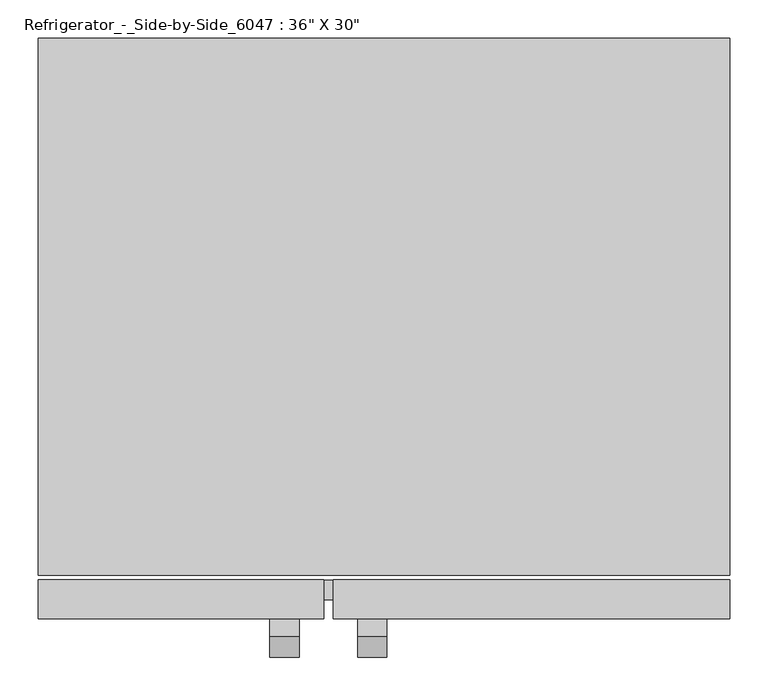
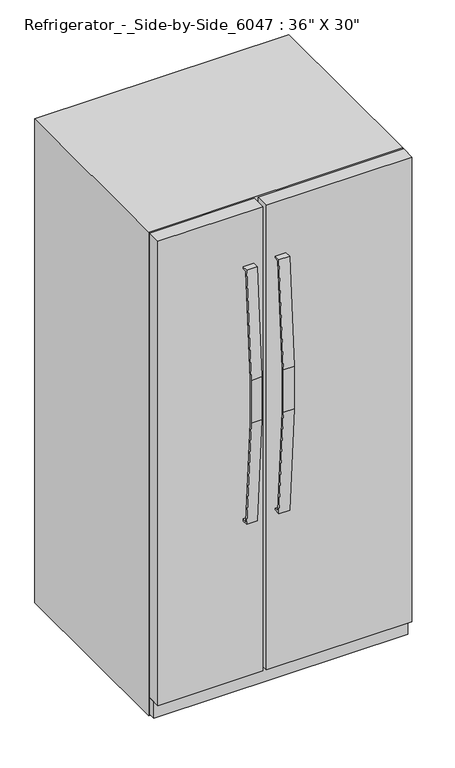
"""IFC4 building model written with IfcOpenShell, lengths in millimetres: proxy geometry."""

import ifcopenshell
import ifcopenshell.guid

model = None  # the IFC model being written
_history = None  # IfcOwnerHistory: only IFC2X3 demands one
_inside = {}  # id of a spatial element -> (the spatial element, [elements in it])
_under = {}  # id of a project, library or spatial element -> (it, [spatial elements below it])
_declared = {}  # id of a project -> (the project, [libraries it declares])
_typed = {}  # id of a type object -> (the type object, [elements of that type])
_made_of = {}  # id of a material, layer set ... -> (it, [elements and type objects made of it])


def new_model(schema):
    """Start an empty IFC model of exactly this schema.

    Asked for "IFC4X3", IfcOpenShell would pick the latest addendum, in which some entities
    have other attributes; the version numbers below select the first issue.
    IFC2X3 requires an IfcOwnerHistory on every rooted entity: one is made here for all.
    """
    global model, _history
    if schema == "IFC4X3":
        model = ifcopenshell.file(schema_version=(4, 3, 0, 0))
    else:
        model = ifcopenshell.file(schema=schema)
    _inside.clear()
    _under.clear()
    _declared.clear()
    _typed.clear()
    _made_of.clear()
    _history = None
    if model.schema == "IFC2X3":
        org = make("IfcOrganization", Name="unknown")
        user = make(
            "IfcPersonAndOrganization",
            ThePerson=make("IfcPerson", FamilyName="unknown"),
            TheOrganization=org,
        )
        app = make(
            "IfcApplication",
            ApplicationDeveloper=org,
            Version="unknown",
            ApplicationFullName="unknown",
            ApplicationIdentifier="unknown",
        )
        _history = make(
            "IfcOwnerHistory",
            OwningUser=user,
            OwningApplication=app,
            ChangeAction="ADDED",
            CreationDate=0,
        )
    return model


def make(cls, **values):
    """One entity of the class cls with the attributes given. An attribute that is None is left unset."""
    return model.create_entity(
        cls, **{name: value for name, value in values.items() if value is not None}
    )


def rooted(cls, **values):
    """An entity with a GlobalId (a new one), such as an element, a storey or a relation."""
    return make(cls, GlobalId=ifcopenshell.guid.new(), OwnerHistory=_history, **values)


def si_unit(unit_type, name, prefix=None):
    """IfcSIUnit, for example si_unit("LENGTHUNIT", "METRE", prefix="MILLI")."""
    return make("IfcSIUnit", UnitType=unit_type, Prefix=prefix, Name=name)


def assignment(units):
    """IfcUnitAssignment: the units of a project."""
    return None if units is None else make("IfcUnitAssignment", Units=units)


def point(xyz):
    """IfcCartesianPoint."""
    return None if xyz is None else make("IfcCartesianPoint", Coordinates=xyz)


def direction(xyz):
    """IfcDirection."""
    return None if xyz is None else make("IfcDirection", DirectionRatios=xyz)


def frame(location, z_axis=None, x_axis=None):
    """IfcAxis2Placement3D, a coordinate frame: its origin and axes. An axis left out is left unset."""
    return make(
        "IfcAxis2Placement3D",
        Location=point(location),
        Axis=direction(z_axis),
        RefDirection=direction(x_axis),
    )


def origin():
    """The frame at (0, 0, 0) with its axes left unset."""
    return frame((0.0, 0.0, 0.0))


def origin_with_axes():
    """The frame at (0, 0, 0) with the z axis (0, 0, 1) and the x axis (1, 0, 0) written out."""
    return frame((0.0, 0.0, 0.0), z_axis=(0.0, 0.0, 1.0), x_axis=(1.0, 0.0, 0.0))


def place(relative_to, where):
    """IfcLocalPlacement: puts the frame where relative to a parent placement (None: the world)."""
    return make(
        "IfcLocalPlacement", PlacementRelTo=relative_to, RelativePlacement=where
    )


def context(
    kind, dimensions, precision=None, world=None, true_north=None, identifier=None
):
    """IfcGeometricRepresentationContext, for example the 3D "Model" context."""
    return make(
        "IfcGeometricRepresentationContext",
        ContextIdentifier=identifier,
        ContextType=kind,
        CoordinateSpaceDimension=dimensions,
        Precision=precision,
        WorldCoordinateSystem=world,
        TrueNorth=true_north,
    )


def project(units=None, contexts=None):
    """IfcProject with its units and contexts."""
    return rooted(
        "IfcProject",
        Name="project",
        RepresentationContexts=contexts,
        UnitsInContext=assignment(units),
    )


def spatial(cls, under=None, at=None, **own):
    """A site, building, storey or space (cls), placed at a placement, below another one or the project."""
    s = rooted(cls, ObjectPlacement=at, **own)
    if under is not None:
        _under.setdefault(under.id(), (under, []))[1].append(s)
    return s


def polyline(points):
    """IfcPolyline through the points."""
    return make("IfcPolyline", Points=[point(p) for p in points])


def outline(outer, holes=None, kind="AREA"):
    """IfcArbitraryClosedProfileDef: a profile drawn as a closed curve; with holes, ...WithVoids."""
    if holes is None:
        return make("IfcArbitraryClosedProfileDef", ProfileType=kind, OuterCurve=outer)
    return make(
        "IfcArbitraryProfileDefWithVoids",
        ProfileType=kind,
        OuterCurve=outer,
        InnerCurves=holes,
    )


def extrude(swept, where, along, depth):
    """IfcExtrudedAreaSolid: the profile swept, set in the frame where, extruded along a direction by depth."""
    return make(
        "IfcExtrudedAreaSolid",
        SweptArea=swept,
        Position=where,
        ExtrudedDirection=direction(along),
        Depth=depth,
    )


def shape(context_of_items, identifier, shape_type, items):
    """IfcShapeRepresentation: the items that make up one representation, for example the "Body"."""
    return make(
        "IfcShapeRepresentation",
        ContextOfItems=context_of_items,
        RepresentationIdentifier=identifier,
        RepresentationType=shape_type,
        Items=items,
    )


def source(mapping_origin, context_of_items, identifier, shape_type, items):
    """IfcRepresentationMap: a shape defined once, which mapped items show again and again."""
    return make(
        "IfcRepresentationMap",
        MappingOrigin=mapping_origin,
        MappedRepresentation=shape(context_of_items, identifier, shape_type, items),
    )


def transform(
    local_origin,
    x_axis=None,
    y_axis=None,
    z_axis=None,
    scale=None,
    scale2=None,
    scale3=None,
    uniform=True,
):
    """IfcCartesianTransformationOperator3D, or its non-uniform kind. x_axis, y_axis, z_axis: its Axis1, 2, 3."""
    if uniform:
        return make(
            "IfcCartesianTransformationOperator3D",
            Axis1=direction(x_axis),
            Axis2=direction(y_axis),
            LocalOrigin=point(local_origin),
            Scale=scale,
            Axis3=direction(z_axis),
        )
    return make(
        "IfcCartesianTransformationOperator3DnonUniform",
        Axis1=direction(x_axis),
        Axis2=direction(y_axis),
        LocalOrigin=point(local_origin),
        Scale=scale,
        Axis3=direction(z_axis),
        Scale2=scale2,
        Scale3=scale3,
    )


def mapped(mapping_source, mapping_target):
    """IfcMappedItem: shows the shape of a source again, moved by a transform."""
    return make(
        "IfcMappedItem", MappingSource=mapping_source, MappingTarget=mapping_target
    )


def made_of(thing, what):
    """Note that an element or type object is made of a material, layer set ...; save() writes the relation."""
    if what is not None:
        _made_of.setdefault(what.id(), (what, []))[1].append(thing)
    return thing


def element(
    cls,
    number,
    at=None,
    inside=None,
    cuts=None,
    type_object=None,
    material=None,
    context=None,
    identifier="Body",
    shape_type=None,
    held_by="IfcProductDefinitionShape",
    body=None,
    shapes=None,
    **own,
):
    """One element of the class cls, such as IfcWall. Its Tag is "e" and its number.

    at: its placement. inside: the storey or other place that contains it. cuts: it is an
    opening in that element (IfcRelVoidsElement). A single representation is given by context,
    identifier, shape_type and body (its items); several are given by shapes. held_by: the class
    of the entity that holds the representations. save() writes the other relations.
    """
    e = rooted(cls, Tag="e%d" % number, ObjectPlacement=at, **own)
    if body is not None:
        shapes = [shape(context, identifier, shape_type, body)]
    if shapes is not None:
        e.Representation = make(held_by, Representations=shapes)
    if inside is not None:
        _inside.setdefault(inside.id(), (inside, []))[1].append(e)
    if cuts is not None:
        rooted(
            "IfcRelVoidsElement", RelatingBuildingElement=cuts, RelatedOpeningElement=e
        )
    if type_object is not None:
        _typed.setdefault(type_object.id(), (type_object, []))[1].append(e)
    return made_of(e, material)


def aggregate(whole, parts):
    """IfcRelAggregates: a whole, such as a stair, and the parts it consists of."""
    return rooted("IfcRelAggregates", RelatingObject=whole, RelatedObjects=parts)


def save(model, path):
    """Write the relations noted so far, then the file.

    IfcRelAggregates (storeys below a building ...), IfcRelContainedInSpatialStructure (elements
    in a storey), IfcRelDefinesByType, IfcRelAssociatesMaterial and IfcRelDeclares: one each for
    every whole, place, type object, material and project.
    """
    for whole, parts in _under.values():
        aggregate(whole, parts)
    for where, things in _inside.values():
        rooted(
            "IfcRelContainedInSpatialStructure",
            RelatedElements=things,
            RelatingStructure=where,
        )
    for kind, things in _typed.values():
        rooted("IfcRelDefinesByType", RelatedObjects=things, RelatingType=kind)
    for what, things in _made_of.values():
        rooted("IfcRelAssociatesMaterial", RelatedObjects=things, RelatingMaterial=what)
    for by, libraries in _declared.values():
        rooted("IfcRelDeclares", RelatingContext=by, RelatedDefinitions=libraries)
    model.write(path)


def proxy_32d0ea93(model_context):
    return source(origin(), model_context, "Body", "SweptSolid", [
        extrude(outline(polyline([(-440.1260285, 1226.3027548), (-440.1260285, 1065.4342469), (-412.6473987, 672.4715334), (-395.6760285, 672.4715334), (-395.6760285, 666.1370017), (-418.5699512, 666.1370017), (-446.4760285, 1065.2125), (-446.4760285, 1226.5245017), (-418.5699512, 1625.6), (-395.6760285, 1625.6), (-395.6760285, 1619.2654683), (-412.6473987, 1619.2654683), (-440.1260285, 1226.3027548)])), frame((-149.8915957, 0.0, 0.0), z_axis=(1.0, 0.0, 0.0), x_axis=(0.0, 1.0, 0.0)), (0.0, 0.0, 1.0), 38.4332978),
        extrude(outline(polyline([(-440.1260285, 1226.3027548), (-440.1260285, 1065.4342469), (-412.6473987, 672.4715334), (-395.6760285, 672.4715334), (-395.6760285, 666.1370017), (-418.5699512, 666.1370017), (-446.4760285, 1065.2125), (-446.4760285, 1226.5245017), (-418.5699512, 1625.6), (-395.6760285, 1625.6), (-395.6760285, 1619.2654683), (-412.6473987, 1619.2654683), (-440.1260285, 1226.3027548)])), frame((-34.5917022, 0.0, 0.0), z_axis=(1.0, 0.0, 0.0), x_axis=(0.0, 1.0, 0.0)), (0.0, 0.0, 1.0), 38.4332978),
        extrude(outline(polyline([(454.025, -344.8760285), (454.025, -370.2760285), (-454.025, -370.2760285), (-454.025, -344.8760285), (454.025, -344.8760285)])), frame((0.0, 0.0, 9.3816357), z_axis=(0.0, 0.0, 1.0), x_axis=(1.0, 0.0, 0.0)), (0.0, 0.0, 1.0), 63.5),
        extrude(outline(polyline([(454.025, 366.3239715), (454.025, -338.5260285), (-454.025, -338.5260285), (-454.025, 366.3239715), (454.025, 366.3239715)])), origin_with_axes(), (0.0, 0.0, 1.0), 1828.8),
        extrude(outline(polyline([(-79.375, -395.6760285), (-454.025, -395.6760285), (-454.025, -344.8760285), (-79.375, -344.8760285), (-79.375, -395.6760285)])), frame((0.0, 0.0, 72.8816357), z_axis=(0.0, 0.0, 1.0), x_axis=(1.0, 0.0, 0.0)), (0.0, 0.0, 1.0), 1755.9183643),
        extrude(outline(polyline([(454.025, -395.6760285), (-66.675, -395.6760285), (-66.675, -344.8760285), (454.025, -344.8760285), (454.025, -395.6760285)])), frame((0.0, 0.0, 72.8816357), z_axis=(0.0, 0.0, 1.0), x_axis=(1.0, 0.0, 0.0)), (0.0, 0.0, 1.0), 1755.9183643),
    ])


if __name__ == "__main__":
    model = new_model("IFC4")
    model_context = context("Model", 3, world=origin())
    ifc_project = project(units=[si_unit("LENGTHUNIT", "METRE", prefix="MILLI")], contexts=[model_context])
    site = spatial("IfcSite", under=ifc_project)
    building = spatial("IfcBuilding", under=site)
    placement = place(None, origin())
    proxy_shape = proxy_32d0ea93(model_context)
    element("IfcBuildingElementProxy", 1, Name="Refrigerator_-_Side-by-Side_6047 : 36\" X 30\"", ObjectType="Refrigerator_-_Side-by-Side_6047 : 36\" X 30\"", at=placement, inside=building, context=model_context, shape_type="MappedRepresentation", body=[
        mapped(proxy_shape, transform((0.0, 0.0, 0.0), x_axis=(1.0, 0.0, 0.0), y_axis=(0.0, 1.0, 0.0), z_axis=(0.0, 0.0, 1.0))),
    ])
    save(model, "model.ifc")

# Revit data of these elements
# Type "Refrigerator_-_Side-by-Side_6047 : 36\" X 30\""
#   Label = "REF."
#   Assembly Code = "E1090400"
#   Depth = 2' - 6"
#   Handle = 0' - 1 1/2"
#   Height = 6' - 0"
#   Rear Clearance = 0' - 2"
#   Top Door Height = 1' - 8"
#   Width = 2' - 11 3/4"
#   Base Material = none
#   Material = none
